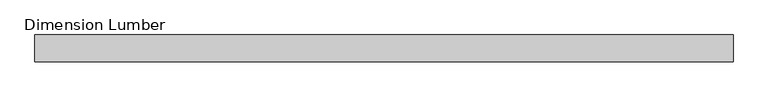
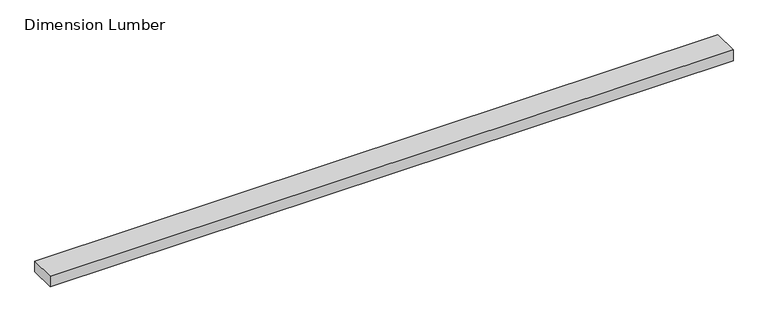
"""IFC4 building model written with IfcOpenShell, lengths in millimetres: beam geometry, Dimension Lumber : Top Supporting Lumbers."""

import ifcopenshell
import ifcopenshell.guid

model = None  # the IFC model being written
_history = None  # IfcOwnerHistory: only IFC2X3 demands one
_inside = {}  # id of a spatial element -> (the spatial element, [elements in it])
_under = {}  # id of a project, library or spatial element -> (it, [spatial elements below it])
_declared = {}  # id of a project -> (the project, [libraries it declares])
_typed = {}  # id of a type object -> (the type object, [elements of that type])
_made_of = {}  # id of a material, layer set ... -> (it, [elements and type objects made of it])


def new_model(schema):
    """Start an empty IFC model of exactly this schema.

    Asked for "IFC4X3", IfcOpenShell would pick the latest addendum, in which some entities
    have other attributes; the version numbers below select the first issue.
    IFC2X3 requires an IfcOwnerHistory on every rooted entity: one is made here for all.
    """
    global model, _history
    if schema == "IFC4X3":
        model = ifcopenshell.file(schema_version=(4, 3, 0, 0))
    else:
        model = ifcopenshell.file(schema=schema)
    _inside.clear()
    _under.clear()
    _declared.clear()
    _typed.clear()
    _made_of.clear()
    _history = None
    if model.schema == "IFC2X3":
        org = make("IfcOrganization", Name="unknown")
        user = make(
            "IfcPersonAndOrganization",
            ThePerson=make("IfcPerson", FamilyName="unknown"),
            TheOrganization=org,
        )
        app = make(
            "IfcApplication",
            ApplicationDeveloper=org,
            Version="unknown",
            ApplicationFullName="unknown",
            ApplicationIdentifier="unknown",
        )
        _history = make(
            "IfcOwnerHistory",
            OwningUser=user,
            OwningApplication=app,
            ChangeAction="ADDED",
            CreationDate=0,
        )
    return model


def make(cls, **values):
    """One entity of the class cls with the attributes given. An attribute that is None is left unset."""
    return model.create_entity(
        cls, **{name: value for name, value in values.items() if value is not None}
    )


def rooted(cls, **values):
    """An entity with a GlobalId (a new one), such as an element, a storey or a relation."""
    return make(cls, GlobalId=ifcopenshell.guid.new(), OwnerHistory=_history, **values)


def si_unit(unit_type, name, prefix=None):
    """IfcSIUnit, for example si_unit("LENGTHUNIT", "METRE", prefix="MILLI")."""
    return make("IfcSIUnit", UnitType=unit_type, Prefix=prefix, Name=name)


def assignment(units):
    """IfcUnitAssignment: the units of a project."""
    return None if units is None else make("IfcUnitAssignment", Units=units)


def point(xyz):
    """IfcCartesianPoint."""
    return None if xyz is None else make("IfcCartesianPoint", Coordinates=xyz)


def direction(xyz):
    """IfcDirection."""
    return None if xyz is None else make("IfcDirection", DirectionRatios=xyz)


def frame(location, z_axis=None, x_axis=None):
    """IfcAxis2Placement3D, a coordinate frame: its origin and axes. An axis left out is left unset."""
    return make(
        "IfcAxis2Placement3D",
        Location=point(location),
        Axis=direction(z_axis),
        RefDirection=direction(x_axis),
    )


def origin():
    """The frame at (0, 0, 0) with its axes left unset."""
    return frame((0.0, 0.0, 0.0))


def place(relative_to, where):
    """IfcLocalPlacement: puts the frame where relative to a parent placement (None: the world)."""
    return make(
        "IfcLocalPlacement", PlacementRelTo=relative_to, RelativePlacement=where
    )


def context(
    kind, dimensions, precision=None, world=None, true_north=None, identifier=None
):
    """IfcGeometricRepresentationContext, for example the 3D "Model" context."""
    return make(
        "IfcGeometricRepresentationContext",
        ContextIdentifier=identifier,
        ContextType=kind,
        CoordinateSpaceDimension=dimensions,
        Precision=precision,
        WorldCoordinateSystem=world,
        TrueNorth=true_north,
    )


def project(units=None, contexts=None):
    """IfcProject with its units and contexts."""
    return rooted(
        "IfcProject",
        Name="project",
        RepresentationContexts=contexts,
        UnitsInContext=assignment(units),
    )


def spatial(cls, under=None, at=None, **own):
    """A site, building, storey or space (cls), placed at a placement, below another one or the project."""
    s = rooted(cls, ObjectPlacement=at, **own)
    if under is not None:
        _under.setdefault(under.id(), (under, []))[1].append(s)
    return s


def polyline(points):
    """IfcPolyline through the points."""
    return make("IfcPolyline", Points=[point(p) for p in points])


def outline(outer, holes=None, kind="AREA"):
    """IfcArbitraryClosedProfileDef: a profile drawn as a closed curve; with holes, ...WithVoids."""
    if holes is None:
        return make("IfcArbitraryClosedProfileDef", ProfileType=kind, OuterCurve=outer)
    return make(
        "IfcArbitraryProfileDefWithVoids",
        ProfileType=kind,
        OuterCurve=outer,
        InnerCurves=holes,
    )


def extrude(swept, where, along, depth):
    """IfcExtrudedAreaSolid: the profile swept, set in the frame where, extruded along a direction by depth."""
    return make(
        "IfcExtrudedAreaSolid",
        SweptArea=swept,
        Position=where,
        ExtrudedDirection=direction(along),
        Depth=depth,
    )


def shape(context_of_items, identifier, shape_type, items):
    """IfcShapeRepresentation: the items that make up one representation, for example the "Body"."""
    return make(
        "IfcShapeRepresentation",
        ContextOfItems=context_of_items,
        RepresentationIdentifier=identifier,
        RepresentationType=shape_type,
        Items=items,
    )


def source(mapping_origin, context_of_items, identifier, shape_type, items):
    """IfcRepresentationMap: a shape defined once, which mapped items show again and again."""
    return make(
        "IfcRepresentationMap",
        MappingOrigin=mapping_origin,
        MappedRepresentation=shape(context_of_items, identifier, shape_type, items),
    )


def transform(
    local_origin,
    x_axis=None,
    y_axis=None,
    z_axis=None,
    scale=None,
    scale2=None,
    scale3=None,
    uniform=True,
):
    """IfcCartesianTransformationOperator3D, or its non-uniform kind. x_axis, y_axis, z_axis: its Axis1, 2, 3."""
    if uniform:
        return make(
            "IfcCartesianTransformationOperator3D",
            Axis1=direction(x_axis),
            Axis2=direction(y_axis),
            LocalOrigin=point(local_origin),
            Scale=scale,
            Axis3=direction(z_axis),
        )
    return make(
        "IfcCartesianTransformationOperator3DnonUniform",
        Axis1=direction(x_axis),
        Axis2=direction(y_axis),
        LocalOrigin=point(local_origin),
        Scale=scale,
        Axis3=direction(z_axis),
        Scale2=scale2,
        Scale3=scale3,
    )


def mapped(mapping_source, mapping_target):
    """IfcMappedItem: shows the shape of a source again, moved by a transform."""
    return make(
        "IfcMappedItem", MappingSource=mapping_source, MappingTarget=mapping_target
    )


def made_of(thing, what):
    """Note that an element or type object is made of a material, layer set ...; save() writes the relation."""
    if what is not None:
        _made_of.setdefault(what.id(), (what, []))[1].append(thing)
    return thing


def element(
    cls,
    number,
    at=None,
    inside=None,
    cuts=None,
    type_object=None,
    material=None,
    context=None,
    identifier="Body",
    shape_type=None,
    held_by="IfcProductDefinitionShape",
    body=None,
    shapes=None,
    **own,
):
    """One element of the class cls, such as IfcWall. Its Tag is "e" and its number.

    at: its placement. inside: the storey or other place that contains it. cuts: it is an
    opening in that element (IfcRelVoidsElement). A single representation is given by context,
    identifier, shape_type and body (its items); several are given by shapes. held_by: the class
    of the entity that holds the representations. save() writes the other relations.
    """
    e = rooted(cls, Tag="e%d" % number, ObjectPlacement=at, **own)
    if body is not None:
        shapes = [shape(context, identifier, shape_type, body)]
    if shapes is not None:
        e.Representation = make(held_by, Representations=shapes)
    if inside is not None:
        _inside.setdefault(inside.id(), (inside, []))[1].append(e)
    if cuts is not None:
        rooted(
            "IfcRelVoidsElement", RelatingBuildingElement=cuts, RelatedOpeningElement=e
        )
    if type_object is not None:
        _typed.setdefault(type_object.id(), (type_object, []))[1].append(e)
    return made_of(e, material)


def aggregate(whole, parts):
    """IfcRelAggregates: a whole, such as a stair, and the parts it consists of."""
    return rooted("IfcRelAggregates", RelatingObject=whole, RelatedObjects=parts)


def save(model, path):
    """Write the relations noted so far, then the file.

    IfcRelAggregates (storeys below a building ...), IfcRelContainedInSpatialStructure (elements
    in a storey), IfcRelDefinesByType, IfcRelAssociatesMaterial and IfcRelDeclares: one each for
    every whole, place, type object, material and project.
    """
    for whole, parts in _under.values():
        aggregate(whole, parts)
    for where, things in _inside.values():
        rooted(
            "IfcRelContainedInSpatialStructure",
            RelatedElements=things,
            RelatingStructure=where,
        )
    for kind, things in _typed.values():
        rooted("IfcRelDefinesByType", RelatedObjects=things, RelatingType=kind)
    for what, things in _made_of.values():
        rooted("IfcRelAssociatesMaterial", RelatedObjects=things, RelatingMaterial=what)
    for by, libraries in _declared.values():
        rooted("IfcRelDeclares", RelatingContext=by, RelatedDefinitions=libraries)
    model.write(path)


def dimension_lumber_c20748c8(model_context):
    return source(origin(), model_context, "Body", "SweptSolid", [
        extrude(outline(polyline([(1155.7, 44.45), (1155.7, -44.45), (-1155.7, -44.45), (-1155.7, 44.45), (1155.7, 44.45)])), frame((0.0, 0.0, -19.05), z_axis=(0.0, 0.0, 1.0), x_axis=(1.0, 0.0, 0.0)), (0.0, 0.0, 1.0), 38.1),
    ])


if __name__ == "__main__":
    model = new_model("IFC4")
    model_context = context("Model", 3, world=origin())
    ifc_project = project(units=[si_unit("LENGTHUNIT", "METRE", prefix="MILLI")], contexts=[model_context])
    site = spatial("IfcSite", under=ifc_project)
    building = spatial("IfcBuilding", under=site)
    placement = place(None, origin())
    dimension_lumber_shape = dimension_lumber_c20748c8(model_context)
    element("IfcBeam", 1, ObjectType="Dimension Lumber : Top Supporting Lumbers", at=placement, inside=building, context=model_context, shape_type="MappedRepresentation", body=[
        mapped(dimension_lumber_shape, transform((0.0, 0.0, 0.0), x_axis=(1.0, 0.0, 0.0), y_axis=(0.0, 1.0, 0.0), z_axis=(0.0, 0.0, 1.0))),
    ])
    save(model, "model.ifc")

# Revit data of these elements
# Type "Dimension Lumber : Top Supporting Lumbers"
#   Assembly Code = "B10"
#   A = 0.0364583 SF
#   Length [instance default] = 5' - 0"
#   b = 0' - 3 1/2"
#   d = 0' - 1 1/2"
#   Structural Material [instance default] = Softwood, Lumber
# Element 1 (IfcBeam, "Dimension Lumber : Top Supporting Lumbers")
#   Structural Material = Douglas Fir #2
#   Materials on its faces: "Douglas Fir #2"
# Materials
#   "Softwood, Lumber": class "Wood", colour RGB 223 192 134, transparency 0, Description = "Pinus Echinata", Cost = 0
#   "Douglas Fir #2": class "Wood", colour RGB 223 192 134, transparency 0, Description = "Pinus Echinata", Cost = 0
